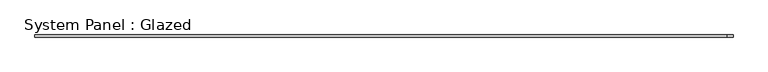
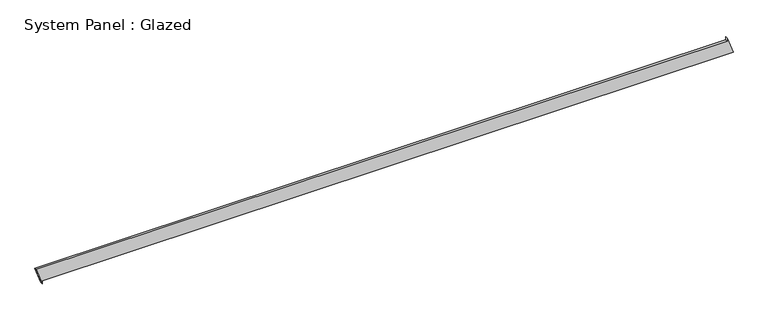
"""IFC4 building model written with IfcOpenShell, lengths in millimetres: plate geometry, System Panel : Glazed."""

import ifcopenshell
import ifcopenshell.guid

model = None  # the IFC model being written
_history = None  # IfcOwnerHistory: only IFC2X3 demands one
_inside = {}  # id of a spatial element -> (the spatial element, [elements in it])
_under = {}  # id of a project, library or spatial element -> (it, [spatial elements below it])
_declared = {}  # id of a project -> (the project, [libraries it declares])
_typed = {}  # id of a type object -> (the type object, [elements of that type])
_made_of = {}  # id of a material, layer set ... -> (it, [elements and type objects made of it])


def new_model(schema):
    """Start an empty IFC model of exactly this schema.

    Asked for "IFC4X3", IfcOpenShell would pick the latest addendum, in which some entities
    have other attributes; the version numbers below select the first issue.
    IFC2X3 requires an IfcOwnerHistory on every rooted entity: one is made here for all.
    """
    global model, _history
    if schema == "IFC4X3":
        model = ifcopenshell.file(schema_version=(4, 3, 0, 0))
    else:
        model = ifcopenshell.file(schema=schema)
    _inside.clear()
    _under.clear()
    _declared.clear()
    _typed.clear()
    _made_of.clear()
    _history = None
    if model.schema == "IFC2X3":
        org = make("IfcOrganization", Name="unknown")
        user = make(
            "IfcPersonAndOrganization",
            ThePerson=make("IfcPerson", FamilyName="unknown"),
            TheOrganization=org,
        )
        app = make(
            "IfcApplication",
            ApplicationDeveloper=org,
            Version="unknown",
            ApplicationFullName="unknown",
            ApplicationIdentifier="unknown",
        )
        _history = make(
            "IfcOwnerHistory",
            OwningUser=user,
            OwningApplication=app,
            ChangeAction="ADDED",
            CreationDate=0,
        )
    return model


def make(cls, **values):
    """One entity of the class cls with the attributes given. An attribute that is None is left unset."""
    return model.create_entity(
        cls, **{name: value for name, value in values.items() if value is not None}
    )


def rooted(cls, **values):
    """An entity with a GlobalId (a new one), such as an element, a storey or a relation."""
    return make(cls, GlobalId=ifcopenshell.guid.new(), OwnerHistory=_history, **values)


def si_unit(unit_type, name, prefix=None):
    """IfcSIUnit, for example si_unit("LENGTHUNIT", "METRE", prefix="MILLI")."""
    return make("IfcSIUnit", UnitType=unit_type, Prefix=prefix, Name=name)


def assignment(units):
    """IfcUnitAssignment: the units of a project."""
    return None if units is None else make("IfcUnitAssignment", Units=units)


def point(xyz):
    """IfcCartesianPoint."""
    return None if xyz is None else make("IfcCartesianPoint", Coordinates=xyz)


def direction(xyz):
    """IfcDirection."""
    return None if xyz is None else make("IfcDirection", DirectionRatios=xyz)


def frame(location, z_axis=None, x_axis=None):
    """IfcAxis2Placement3D, a coordinate frame: its origin and axes. An axis left out is left unset."""
    return make(
        "IfcAxis2Placement3D",
        Location=point(location),
        Axis=direction(z_axis),
        RefDirection=direction(x_axis),
    )


def origin():
    """The frame at (0, 0, 0) with its axes left unset."""
    return frame((0.0, 0.0, 0.0))


def place(relative_to, where):
    """IfcLocalPlacement: puts the frame where relative to a parent placement (None: the world)."""
    return make(
        "IfcLocalPlacement", PlacementRelTo=relative_to, RelativePlacement=where
    )


def context(
    kind, dimensions, precision=None, world=None, true_north=None, identifier=None
):
    """IfcGeometricRepresentationContext, for example the 3D "Model" context."""
    return make(
        "IfcGeometricRepresentationContext",
        ContextIdentifier=identifier,
        ContextType=kind,
        CoordinateSpaceDimension=dimensions,
        Precision=precision,
        WorldCoordinateSystem=world,
        TrueNorth=true_north,
    )


def project(units=None, contexts=None):
    """IfcProject with its units and contexts."""
    return rooted(
        "IfcProject",
        Name="project",
        RepresentationContexts=contexts,
        UnitsInContext=assignment(units),
    )


def spatial(cls, under=None, at=None, **own):
    """A site, building, storey or space (cls), placed at a placement, below another one or the project."""
    s = rooted(cls, ObjectPlacement=at, **own)
    if under is not None:
        _under.setdefault(under.id(), (under, []))[1].append(s)
    return s


def polyline(points):
    """IfcPolyline through the points."""
    return make("IfcPolyline", Points=[point(p) for p in points])


def outline(outer, holes=None, kind="AREA"):
    """IfcArbitraryClosedProfileDef: a profile drawn as a closed curve; with holes, ...WithVoids."""
    if holes is None:
        return make("IfcArbitraryClosedProfileDef", ProfileType=kind, OuterCurve=outer)
    return make(
        "IfcArbitraryProfileDefWithVoids",
        ProfileType=kind,
        OuterCurve=outer,
        InnerCurves=holes,
    )


def extrude(swept, where, along, depth):
    """IfcExtrudedAreaSolid: the profile swept, set in the frame where, extruded along a direction by depth."""
    return make(
        "IfcExtrudedAreaSolid",
        SweptArea=swept,
        Position=where,
        ExtrudedDirection=direction(along),
        Depth=depth,
    )


def shape(context_of_items, identifier, shape_type, items):
    """IfcShapeRepresentation: the items that make up one representation, for example the "Body"."""
    return make(
        "IfcShapeRepresentation",
        ContextOfItems=context_of_items,
        RepresentationIdentifier=identifier,
        RepresentationType=shape_type,
        Items=items,
    )


def source(mapping_origin, context_of_items, identifier, shape_type, items):
    """IfcRepresentationMap: a shape defined once, which mapped items show again and again."""
    return make(
        "IfcRepresentationMap",
        MappingOrigin=mapping_origin,
        MappedRepresentation=shape(context_of_items, identifier, shape_type, items),
    )


def transform(
    local_origin,
    x_axis=None,
    y_axis=None,
    z_axis=None,
    scale=None,
    scale2=None,
    scale3=None,
    uniform=True,
):
    """IfcCartesianTransformationOperator3D, or its non-uniform kind. x_axis, y_axis, z_axis: its Axis1, 2, 3."""
    if uniform:
        return make(
            "IfcCartesianTransformationOperator3D",
            Axis1=direction(x_axis),
            Axis2=direction(y_axis),
            LocalOrigin=point(local_origin),
            Scale=scale,
            Axis3=direction(z_axis),
        )
    return make(
        "IfcCartesianTransformationOperator3DnonUniform",
        Axis1=direction(x_axis),
        Axis2=direction(y_axis),
        LocalOrigin=point(local_origin),
        Scale=scale,
        Axis3=direction(z_axis),
        Scale2=scale2,
        Scale3=scale3,
    )


def mapped(mapping_source, mapping_target):
    """IfcMappedItem: shows the shape of a source again, moved by a transform."""
    return make(
        "IfcMappedItem", MappingSource=mapping_source, MappingTarget=mapping_target
    )


def made_of(thing, what):
    """Note that an element or type object is made of a material, layer set ...; save() writes the relation."""
    if what is not None:
        _made_of.setdefault(what.id(), (what, []))[1].append(thing)
    return thing


def element(
    cls,
    number,
    at=None,
    inside=None,
    cuts=None,
    type_object=None,
    material=None,
    context=None,
    identifier="Body",
    shape_type=None,
    held_by="IfcProductDefinitionShape",
    body=None,
    shapes=None,
    **own,
):
    """One element of the class cls, such as IfcWall. Its Tag is "e" and its number.

    at: its placement. inside: the storey or other place that contains it. cuts: it is an
    opening in that element (IfcRelVoidsElement). A single representation is given by context,
    identifier, shape_type and body (its items); several are given by shapes. held_by: the class
    of the entity that holds the representations. save() writes the other relations.
    """
    e = rooted(cls, Tag="e%d" % number, ObjectPlacement=at, **own)
    if body is not None:
        shapes = [shape(context, identifier, shape_type, body)]
    if shapes is not None:
        e.Representation = make(held_by, Representations=shapes)
    if inside is not None:
        _inside.setdefault(inside.id(), (inside, []))[1].append(e)
    if cuts is not None:
        rooted(
            "IfcRelVoidsElement", RelatingBuildingElement=cuts, RelatedOpeningElement=e
        )
    if type_object is not None:
        _typed.setdefault(type_object.id(), (type_object, []))[1].append(e)
    return made_of(e, material)


def aggregate(whole, parts):
    """IfcRelAggregates: a whole, such as a stair, and the parts it consists of."""
    return rooted("IfcRelAggregates", RelatingObject=whole, RelatedObjects=parts)


def save(model, path):
    """Write the relations noted so far, then the file.

    IfcRelAggregates (storeys below a building ...), IfcRelContainedInSpatialStructure (elements
    in a storey), IfcRelDefinesByType, IfcRelAssociatesMaterial and IfcRelDeclares: one each for
    every whole, place, type object, material and project.
    """
    for whole, parts in _under.values():
        aggregate(whole, parts)
    for where, things in _inside.values():
        rooted(
            "IfcRelContainedInSpatialStructure",
            RelatedElements=things,
            RelatingStructure=where,
        )
    for kind, things in _typed.values():
        rooted("IfcRelDefinesByType", RelatedObjects=things, RelatingType=kind)
    for what, things in _made_of.values():
        rooted("IfcRelAssociatesMaterial", RelatedObjects=things, RelatingMaterial=what)
    for by, libraries in _declared.values():
        rooted("IfcRelDeclares", RelatingContext=by, RelatedDefinitions=libraries)
    model.write(path)


def system_panel_glazed_ae9a7b9e(model_context):
    return source(origin(), model_context, "Body", "SweptSolid", [
        extrude(outline(polyline([(0.0, -3958.3929013), (35.3553391, -3958.3929013), (35.3553391, 4028.5329041), (235.1902238, 3958.4993271), (199.8348847, 3958.4995256), (199.7900514, -4028.5329041), (0.0, -3958.3929013)])), frame((0.0, -49.5, 0.0), z_axis=(0.0, 1.0, 0.0), x_axis=(0.0, 0.0, 1.0)), (0.0, 0.0, 1.0), 25.0),
    ])


if __name__ == "__main__":
    model = new_model("IFC4")
    model_context = context("Model", 3, world=origin())
    ifc_project = project(units=[si_unit("LENGTHUNIT", "METRE", prefix="MILLI")], contexts=[model_context])
    site = spatial("IfcSite", under=ifc_project)
    building = spatial("IfcBuilding", under=site)
    placement = place(None, origin())
    system_panel_glazed_shape = system_panel_glazed_ae9a7b9e(model_context)
    element("IfcPlate", 1, ObjectType="System Panel : Glazed", at=placement, inside=building, context=model_context, shape_type="MappedRepresentation", body=[
        mapped(system_panel_glazed_shape, transform((0.0, 0.0, 0.0), x_axis=(1.0, 0.0, 0.0), y_axis=(0.0, 1.0, 0.0), z_axis=(0.0, 0.0, 1.0))),
    ])
    save(model, "model.ifc")

# Revit data of these elements
# Element 1 (IfcPlate, "System Panel : Glazed")
#   Materials on its faces: "Glass"
# Materials
#   "Glass": class "Glass", colour RGB 218 227 224, transparency 0.85, Description = "Soda Lime Glass", Cost = 0
